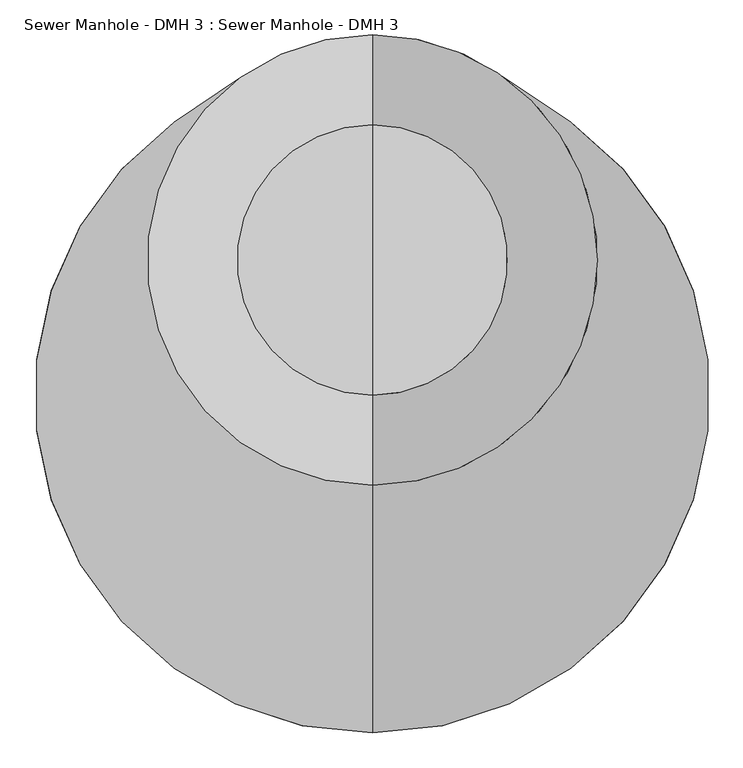
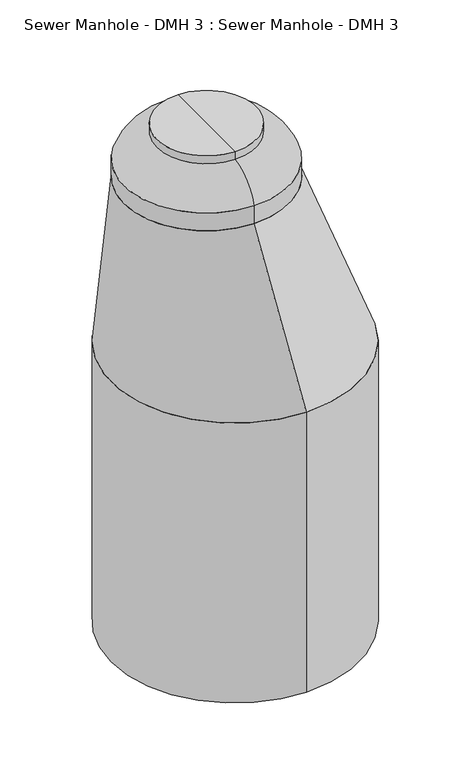
"""IFC4 building model written with IfcOpenShell, lengths in millimetres: proxy geometry, Sewer Manhole - DMH 3 : Sewer Manhole - DMH 3."""

from ifc_helpers import new_model, si_unit, point, frame, origin, place, context, project, spatial, circle_curve, ellipse_curve, trimmed, source, transform, mapped, element, save
from ifc_brep_helpers import plane_surface, cylinder_surface, revolved_surface, spline_surface, advanced_brep


def sewer_manhole_dmh_3_sewer_manhole_dmh_3_05a0183f(model_context):
    return source(origin(), model_context, "Body", "AdvancedBrep", [
        advanced_brep(
        [(0.0, 812.8, 2704.3270774), (0.0, -203.2, 2704.3270774), (0.0, 762.0, 1818.64), (0.0, -762.0, 1818.64)],
        [
            (0, 1, circle_curve(frame((0.0, 304.8, 2704.3270774), z_axis=(0.0, 0.0, 1.0), x_axis=(0.0, 1.0, 0.0)), 508.0)),
            (1, 0, circle_curve(frame((0.0, 304.8, 2704.3270774), z_axis=(0.0, 0.0, 1.0), x_axis=(0.0, 1.0, 0.0)), 508.0)),
            (2, 3, circle_curve(frame((0.0, 0.0, 1818.64), z_axis=(0.0, 0.0, -1.0), x_axis=(0.0, 1.0, 0.0)), 762.0)),
            (3, 2, circle_curve(frame((0.0, 0.0, 1818.64), z_axis=(0.0, 0.0, -1.0), x_axis=(0.0, 1.0, 0.0)), 762.0)),
            (3, 1),
            (0, 2),
        ],
        [
            plane_surface(frame((0.0, 304.8, 2704.3270774), z_axis=(0.0, 0.0, 1.0), x_axis=(1.0, 0.0, 0.0))),
            plane_surface(frame((0.0, 0.0, 1818.64), z_axis=(0.0, 0.0, -1.0), x_axis=(1.0, 0.0, 0.0))),
            spline_surface(2, 1, [[(0.0, 762.0, 1818.64), (0.0, 812.8, 2704.3270774)], [(-762.0, 762.0, 1818.64), (-507.99999999999994, 812.8, 2704.3270774)], [(-762.0, 0.0, 1818.64), (-507.99999999999994, 304.8, 2704.3270774)], [(-762.0, -762.0, 1818.64), (-507.99999999999994, -203.19999999999993, 2704.3270774)], [(0.0, -762.0, 1818.64), (0.0, -203.2, 2704.3270774)]], [3, 2, 3], [2, 2], [0.0, 1.0, 2.0], [0.0, 1.0], weights=[[1.0, 1.0], [0.7071067811865476, 0.7071067811865476], [1.0, 1.0], [0.7071067811865476, 0.7071067811865476], [1.0, 1.0]]),
            spline_surface(2, 1, [[(0.0, -762.0, 1818.64), (0.0, -203.2, 2704.3270774)], [(762.0, -762.0, 1818.64), (508.0, -203.2, 2704.3270774)], [(762.0, 0.0, 1818.64), (508.0, 304.8, 2704.3270774)], [(762.0, 762.0, 1818.64), (508.0, 812.8, 2704.3270774)], [(0.0, 762.0, 1818.64), (0.0, 812.8, 2704.3270774)]], [3, 2, 3], [2, 2], [0.0, 1.0, 2.0], [0.0, 1.0], weights=[[1.0, 1.0], [0.7071067811865476, 0.7071067811865476], [1.0, 1.0], [0.7071067811865476, 0.7071067811865476], [1.0, 1.0]]),
        ],
        [
            (0, [[1, 2]]),
            (1, [[3, 4]]),
            (2, [[-4, 5, -1, 6]]),
            (3, [[-3, -6, -2, -5]]),
        ],
    ),
        advanced_brep(
        [(0.0, -203.2, 2704.3270774), (0.0, 812.8, 2704.3270774), (0.0, 304.8, 2704.3270774), (0.0, -203.2, 2819.4), (0.0, 812.8, 2819.4), (0.0, 0.0, 2997.2), (0.0, 609.6, 2997.2), (0.0, 0.0, 3048.0), (0.0, 609.6, 3048.0), (0.0, 304.8, 3048.0)],
        [
            (0, 1, circle_curve(frame((0.0, 304.8, 2704.3270774), z_axis=(0.0, 0.0, -1.0), x_axis=(0.0, 1.0, 0.0)), 508.0)),
            (1, 2),
            (2, 0),
            (1, 0, circle_curve(frame((0.0, 304.8, 2704.3270774), z_axis=(0.0, 0.0, -1.0), x_axis=(0.0, 1.0, 0.0)), 508.0)),
            (3, 4, circle_curve(frame((0.0, 304.8, 2819.4), z_axis=(0.0, 0.0, -1.0), x_axis=(0.0, 1.0, 0.0)), 508.0)),
            (4, 1),
            (0, 3),
            (4, 3, circle_curve(frame((0.0, 304.8, 2819.4), z_axis=(0.0, 0.0, -1.0), x_axis=(0.0, 1.0, 0.0)), 508.0)),
            (5, 6, circle_curve(frame((0.0, 304.8, 2997.2), z_axis=(0.0, 0.0, -1.0), x_axis=(0.0, 1.0, 0.0)), 304.8)),
            (6, 4, circle_curve(frame((0.0, 564.4539436, 2740.5902213), z_axis=(-1.0, 0.0, 0.0), x_axis=(0.0, -1.0, 0.0)), 260.550849)),
            (3, 5, circle_curve(frame((0.0, 45.1460564, 2740.5902213), z_axis=(-1.0, 0.0, 0.0), x_axis=(0.0, 1.0, 0.0)), 260.550849)),
            (6, 5, circle_curve(frame((0.0, 304.8, 2997.2), z_axis=(0.0, 0.0, -1.0), x_axis=(0.0, 1.0, 0.0)), 304.8)),
            (7, 8, circle_curve(frame((0.0, 304.8, 3048.0), z_axis=(0.0, 0.0, -1.0), x_axis=(0.0, 1.0, 0.0)), 304.8)),
            (8, 6),
            (5, 7),
            (8, 7, circle_curve(frame((0.0, 304.8, 3048.0), z_axis=(0.0, 0.0, -1.0), x_axis=(0.0, 1.0, 0.0)), 304.8)),
            (9, 8),
            (7, 9),
        ],
        [
            plane_surface(frame((0.0, 304.8, 2704.3270774), z_axis=(0.0, 0.0, -1.0), x_axis=(0.0, 1.0, 0.0))),
            cylinder_surface(frame((0.0, 304.8, 2768.6), z_axis=(0.0, 0.0, 1.0), x_axis=(0.0, 1.0, 0.0)), 508.0),
            revolved_surface(trimmed(ellipse_curve(frame((0.0, 564.4539436, 2740.5902213), z_axis=(1.0, 0.0, 0.0), x_axis=(0.0, -1.0, 0.0)), 260.550849, 260.550849), [point((0.0, 812.8, 2819.4))], [point((0.0, 609.6, 2997.2))], True, "CARTESIAN"), (0.0, 304.8, 2768.6), (0.0, 0.0, 1.0)),
            cylinder_surface(frame((0.0, 304.8, 2768.6), z_axis=(0.0, 0.0, 1.0), x_axis=(0.0, 1.0, 0.0)), 304.8),
            plane_surface(frame((0.0, 304.8, 3048.0), z_axis=(0.0, 0.0, 1.0), x_axis=(0.0, 1.0, 0.0))),
        ],
        [
            (0, [[1, 2, 3]]),
            (0, [[4, -3, -2]]),
            (1, [[5, 6, -1, 7]]),
            (1, [[8, -7, -4, -6]]),
            (2, [[9, 10, -5, 11]]),
            (2, [[12, -11, -8, -10]]),
            (3, [[13, 14, -9, 15]]),
            (3, [[16, -15, -12, -14]]),
            (4, [[17, -13, 18]]),
            (4, [[-18, -16, -17]]),
        ],
    ),
        advanced_brep(
        [(0.0, -762.0, 1818.64), (0.0, 762.0, 1818.64), (0.0, 762.0, 0.0), (0.0, -762.0, 0.0), (0.0, 0.0, 0.0), (0.0, 0.0, 1818.64)],
        [
            (0, 1, circle_curve(frame((0.0, 0.0, 1818.64), z_axis=(0.0, 0.0, -1.0), x_axis=(0.0, 1.0, 0.0)), 762.0)),
            (1, 2),
            (2, 3, circle_curve(frame((0.0, 0.0, 0.0), z_axis=(0.0, 0.0, 1.0), x_axis=(0.0, 1.0, 0.0)), 762.0)),
            (3, 0),
            (1, 0, circle_curve(frame((0.0, 0.0, 1818.64), z_axis=(0.0, 0.0, -1.0), x_axis=(0.0, 1.0, 0.0)), 762.0)),
            (3, 2, circle_curve(frame((0.0, 0.0, 0.0), z_axis=(0.0, 0.0, 1.0), x_axis=(0.0, 1.0, 0.0)), 762.0)),
            (2, 4),
            (4, 3),
            (5, 1),
            (0, 5),
        ],
        [
            cylinder_surface(frame((0.0, 0.0, 457.2), z_axis=(0.0, 0.0, 1.0), x_axis=(0.0, 1.0, 0.0)), 762.0),
            plane_surface(frame((0.0, 0.0, 0.0), z_axis=(0.0, 0.0, -1.0), x_axis=(0.0, 1.0, 0.0))),
            plane_surface(frame((0.0, 0.0, 1818.64), z_axis=(0.0, 0.0, 1.0), x_axis=(0.0, 1.0, 0.0))),
        ],
        [
            (0, [[1, 2, 3, 4]]),
            (0, [[5, -4, 6, -2]]),
            (1, [[-3, 7, 8]]),
            (1, [[-6, -8, -7]]),
            (2, [[9, -1, 10]]),
            (2, [[-10, -5, -9]]),
        ],
    ),
    ])


if __name__ == "__main__":
    model = new_model("IFC4")
    model_context = context("Model", 3, world=origin())
    ifc_project = project(units=[si_unit("LENGTHUNIT", "METRE", prefix="MILLI")], contexts=[model_context])
    site = spatial("IfcSite", under=ifc_project)
    building = spatial("IfcBuilding", under=site)
    placement = place(None, origin())
    sewer_manhole_dmh_3_sewer_manhole_dmh_3_shape = sewer_manhole_dmh_3_sewer_manhole_dmh_3_05a0183f(model_context)
    element("IfcBuildingElementProxy", 1, Name="Sewer Manhole - DMH 3 : Sewer Manhole - DMH 3", ObjectType="Sewer Manhole - DMH 3 : Sewer Manhole - DMH 3", at=placement, inside=building, context=model_context, shape_type="MappedRepresentation", body=[
        mapped(sewer_manhole_dmh_3_sewer_manhole_dmh_3_shape, transform((0.0, 0.0, 0.0), x_axis=(1.0, 0.0, 0.0), y_axis=(0.0, 1.0, 0.0), z_axis=(0.0, 0.0, 1.0))),
    ])
    save(model, "model.ifc")

# Revit data of these elements
# Project information
#   TBC Electrician = "ELECTRICIAN HERE"
#   TBC Fire Protection = "FP HERE"
#   TBC Plumber = "PLUMBER HERE"
#   TBC HVAC = "HVAC HERE"
#   TBC Other Company 1 = "MISC COMPANY 1"
#   TBC Other Company 2 = "MISC COMPANY 2"
#   TBC COORDINATOR = "NAME OF VCC"
#   Workset = "Project Info"
#   Project Issue Date = "2010.12.07"
#   Project Status = "Project Status"
#   Client Name = "Owner"
#   Project Address = "111 BOYLSTON STREET, \nBROOKLINE MA"
#   Project Name = "HOMEWOOD SUITES"
#   Project Number = "13381"
